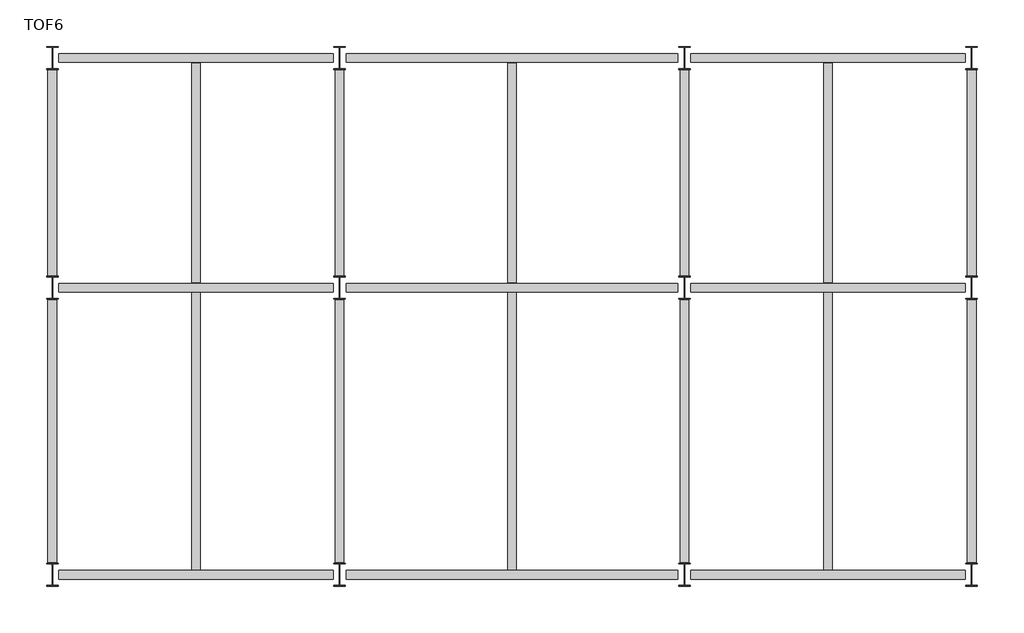
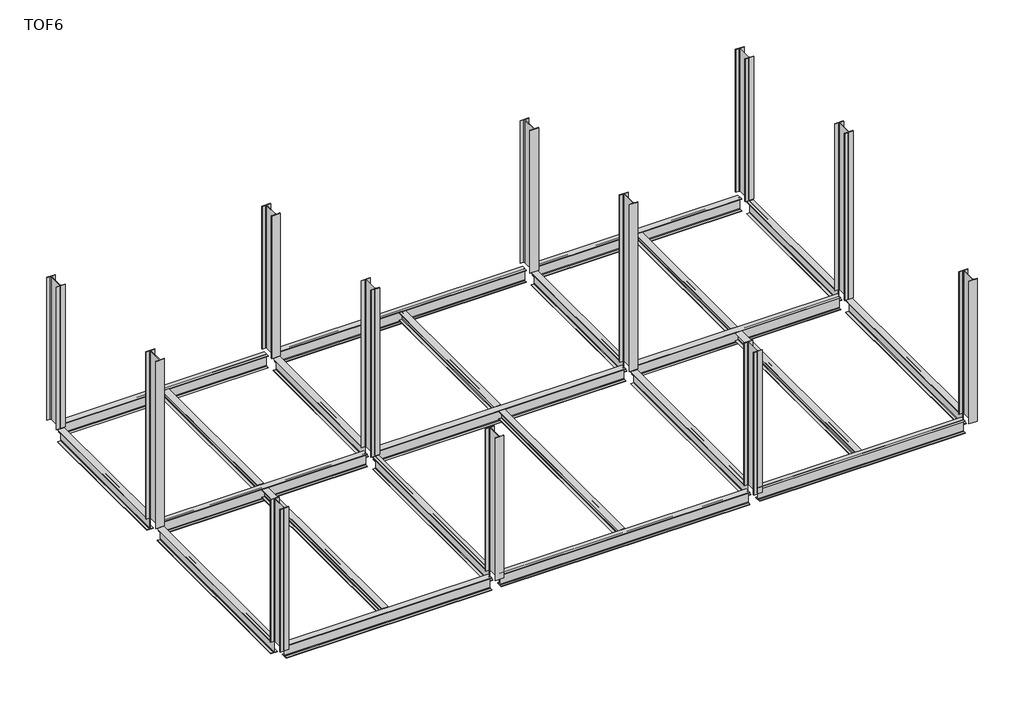
# One storey: 23 beams, 12 columns.
"""IFC4 building model written with IfcOpenShell, lengths in millimetres."""

import ifcopenshell
import ifcopenshell.guid

model = None  # the IFC model being written
_history = None  # IfcOwnerHistory: only IFC2X3 demands one
_inside = {}  # id of a spatial element -> (the spatial element, [elements in it])
_under = {}  # id of a project, library or spatial element -> (it, [spatial elements below it])
_declared = {}  # id of a project -> (the project, [libraries it declares])
_typed = {}  # id of a type object -> (the type object, [elements of that type])
_made_of = {}  # id of a material, layer set ... -> (it, [elements and type objects made of it])


def new_model(schema):
    """Start an empty IFC model of exactly this schema.

    Asked for "IFC4X3", IfcOpenShell would pick the latest addendum, in which some entities
    have other attributes; the version numbers below select the first issue.
    IFC2X3 requires an IfcOwnerHistory on every rooted entity: one is made here for all.
    """
    global model, _history
    if schema == "IFC4X3":
        model = ifcopenshell.file(schema_version=(4, 3, 0, 0))
    else:
        model = ifcopenshell.file(schema=schema)
    _inside.clear()
    _under.clear()
    _declared.clear()
    _typed.clear()
    _made_of.clear()
    _history = None
    if model.schema == "IFC2X3":
        org = make("IfcOrganization", Name="unknown")
        user = make(
            "IfcPersonAndOrganization",
            ThePerson=make("IfcPerson", FamilyName="unknown"),
            TheOrganization=org,
        )
        app = make(
            "IfcApplication",
            ApplicationDeveloper=org,
            Version="unknown",
            ApplicationFullName="unknown",
            ApplicationIdentifier="unknown",
        )
        _history = make(
            "IfcOwnerHistory",
            OwningUser=user,
            OwningApplication=app,
            ChangeAction="ADDED",
            CreationDate=0,
        )
    return model


def make(cls, **values):
    """One entity of the class cls with the attributes given. An attribute that is None is left unset."""
    return model.create_entity(
        cls, **{name: value for name, value in values.items() if value is not None}
    )


def rooted(cls, **values):
    """An entity with a GlobalId (a new one), such as an element, a storey or a relation."""
    return make(cls, GlobalId=ifcopenshell.guid.new(), OwnerHistory=_history, **values)


def si_unit(unit_type, name, prefix=None):
    """IfcSIUnit, for example si_unit("LENGTHUNIT", "METRE", prefix="MILLI")."""
    return make("IfcSIUnit", UnitType=unit_type, Prefix=prefix, Name=name)


def assignment(units):
    """IfcUnitAssignment: the units of a project."""
    return None if units is None else make("IfcUnitAssignment", Units=units)


def point(xyz):
    """IfcCartesianPoint."""
    return None if xyz is None else make("IfcCartesianPoint", Coordinates=xyz)


def direction(xyz):
    """IfcDirection."""
    return None if xyz is None else make("IfcDirection", DirectionRatios=xyz)


def frame(location, z_axis=None, x_axis=None):
    """IfcAxis2Placement3D, a coordinate frame: its origin and axes. An axis left out is left unset."""
    return make(
        "IfcAxis2Placement3D",
        Location=point(location),
        Axis=direction(z_axis),
        RefDirection=direction(x_axis),
    )


def frame_2d(location, x_axis=None):
    """IfcAxis2Placement2D, a coordinate frame in the plane: its origin and x axis."""
    return make(
        "IfcAxis2Placement2D", Location=point(location), RefDirection=direction(x_axis)
    )


def origin():
    """The frame at (0, 0, 0) with its axes left unset."""
    return frame((0.0, 0.0, 0.0))


def place(relative_to, where):
    """IfcLocalPlacement: puts the frame where relative to a parent placement (None: the world)."""
    return make(
        "IfcLocalPlacement", PlacementRelTo=relative_to, RelativePlacement=where
    )


def context(
    kind, dimensions, precision=None, world=None, true_north=None, identifier=None
):
    """IfcGeometricRepresentationContext, for example the 3D "Model" context."""
    return make(
        "IfcGeometricRepresentationContext",
        ContextIdentifier=identifier,
        ContextType=kind,
        CoordinateSpaceDimension=dimensions,
        Precision=precision,
        WorldCoordinateSystem=world,
        TrueNorth=true_north,
    )


def project(units=None, contexts=None):
    """IfcProject with its units and contexts."""
    return rooted(
        "IfcProject",
        Name="project",
        RepresentationContexts=contexts,
        UnitsInContext=assignment(units),
    )


def spatial(cls, under=None, at=None, **own):
    """A site, building, storey or space (cls), placed at a placement, below another one or the project."""
    s = rooted(cls, ObjectPlacement=at, **own)
    if under is not None:
        _under.setdefault(under.id(), (under, []))[1].append(s)
    return s


def polyline(points):
    """IfcPolyline through the points."""
    return make("IfcPolyline", Points=[point(p) for p in points])


def circle_curve(where, radius):
    """IfcCircle in the frame where."""
    return make("IfcCircle", Position=where, Radius=radius)


def trimmed(basis, trim1, trim2, sense, master):
    """IfcTrimmedCurve: the piece of a basis curve between two trims."""
    return make(
        "IfcTrimmedCurve",
        BasisCurve=basis,
        Trim1=trim1,
        Trim2=trim2,
        SenseAgreement=sense,
        MasterRepresentation=master,
    )


def segment(curve, same_sense, transition):
    """IfcCompositeCurveSegment."""
    return make(
        "IfcCompositeCurveSegment",
        Transition=transition,
        SameSense=same_sense,
        ParentCurve=curve,
    )


def composite_curve(segments, self_intersect=None):
    """IfcCompositeCurve: segments joined end to end."""
    return make("IfcCompositeCurve", Segments=segments, SelfIntersect=self_intersect)


def outline(outer, holes=None, kind="AREA"):
    """IfcArbitraryClosedProfileDef: a profile drawn as a closed curve; with holes, ...WithVoids."""
    if holes is None:
        return make("IfcArbitraryClosedProfileDef", ProfileType=kind, OuterCurve=outer)
    return make(
        "IfcArbitraryProfileDefWithVoids",
        ProfileType=kind,
        OuterCurve=outer,
        InnerCurves=holes,
    )


def extrude(swept, where, along, depth):
    """IfcExtrudedAreaSolid: the profile swept, set in the frame where, extruded along a direction by depth."""
    return make(
        "IfcExtrudedAreaSolid",
        SweptArea=swept,
        Position=where,
        ExtrudedDirection=direction(along),
        Depth=depth,
    )


def shape(context_of_items, identifier, shape_type, items):
    """IfcShapeRepresentation: the items that make up one representation, for example the "Body"."""
    return make(
        "IfcShapeRepresentation",
        ContextOfItems=context_of_items,
        RepresentationIdentifier=identifier,
        RepresentationType=shape_type,
        Items=items,
    )


def source(mapping_origin, context_of_items, identifier, shape_type, items):
    """IfcRepresentationMap: a shape defined once, which mapped items show again and again."""
    return make(
        "IfcRepresentationMap",
        MappingOrigin=mapping_origin,
        MappedRepresentation=shape(context_of_items, identifier, shape_type, items),
    )


def transform(
    local_origin,
    x_axis=None,
    y_axis=None,
    z_axis=None,
    scale=None,
    scale2=None,
    scale3=None,
    uniform=True,
):
    """IfcCartesianTransformationOperator3D, or its non-uniform kind. x_axis, y_axis, z_axis: its Axis1, 2, 3."""
    if uniform:
        return make(
            "IfcCartesianTransformationOperator3D",
            Axis1=direction(x_axis),
            Axis2=direction(y_axis),
            LocalOrigin=point(local_origin),
            Scale=scale,
            Axis3=direction(z_axis),
        )
    return make(
        "IfcCartesianTransformationOperator3DnonUniform",
        Axis1=direction(x_axis),
        Axis2=direction(y_axis),
        LocalOrigin=point(local_origin),
        Scale=scale,
        Axis3=direction(z_axis),
        Scale2=scale2,
        Scale3=scale3,
    )


def mapped(mapping_source, mapping_target):
    """IfcMappedItem: shows the shape of a source again, moved by a transform."""
    return make(
        "IfcMappedItem", MappingSource=mapping_source, MappingTarget=mapping_target
    )


def made_of(thing, what):
    """Note that an element or type object is made of a material, layer set ...; save() writes the relation."""
    if what is not None:
        _made_of.setdefault(what.id(), (what, []))[1].append(thing)
    return thing


def element(
    cls,
    number,
    at=None,
    inside=None,
    cuts=None,
    type_object=None,
    material=None,
    context=None,
    identifier="Body",
    shape_type=None,
    held_by="IfcProductDefinitionShape",
    body=None,
    shapes=None,
    **own,
):
    """One element of the class cls, such as IfcWall. Its Tag is "e" and its number.

    at: its placement. inside: the storey or other place that contains it. cuts: it is an
    opening in that element (IfcRelVoidsElement). A single representation is given by context,
    identifier, shape_type and body (its items); several are given by shapes. held_by: the class
    of the entity that holds the representations. save() writes the other relations.
    """
    e = rooted(cls, Tag="e%d" % number, ObjectPlacement=at, **own)
    if body is not None:
        shapes = [shape(context, identifier, shape_type, body)]
    if shapes is not None:
        e.Representation = make(held_by, Representations=shapes)
    if inside is not None:
        _inside.setdefault(inside.id(), (inside, []))[1].append(e)
    if cuts is not None:
        rooted(
            "IfcRelVoidsElement", RelatingBuildingElement=cuts, RelatedOpeningElement=e
        )
    if type_object is not None:
        _typed.setdefault(type_object.id(), (type_object, []))[1].append(e)
    return made_of(e, material)


def aggregate(whole, parts):
    """IfcRelAggregates: a whole, such as a stair, and the parts it consists of."""
    return rooted("IfcRelAggregates", RelatingObject=whole, RelatedObjects=parts)


def save(model, path):
    """Write the relations noted so far, then the file.

    IfcRelAggregates (storeys below a building ...), IfcRelContainedInSpatialStructure (elements
    in a storey), IfcRelDefinesByType, IfcRelAssociatesMaterial and IfcRelDeclares: one each for
    every whole, place, type object, material and project.
    """
    for whole, parts in _under.values():
        aggregate(whole, parts)
    for where, things in _inside.values():
        rooted(
            "IfcRelContainedInSpatialStructure",
            RelatedElements=things,
            RelatingStructure=where,
        )
    for kind, things in _typed.values():
        rooted("IfcRelDefinesByType", RelatedObjects=things, RelatingType=kind)
    for what, things in _made_of.values():
        rooted("IfcRelAssociatesMaterial", RelatedObjects=things, RelatingMaterial=what)
    for by, libraries in _declared.values():
        rooted("IfcRelDeclares", RelatingContext=by, RelatedDefinitions=libraries)
    model.write(path)


def beam_a4a24592(model_context):
    return source(origin(), model_context, "Body", "SweptSolid", [
        extrude(outline(composite_curve([segment(polyline([(75.0, -141.0), (75.0, -150.0), (-75.0, -150.0), (-75.0, -141.0), (-16.25, -141.0)]), True, "CONTINUOUS"), segment(trimmed(circle_curve(frame_2d((-16.25, -128.0)), 13.0), [point((-16.25, -141.0))], [point((-3.25, -128.0))], True, "CARTESIAN"), True, "CONTINUOUS"), segment(polyline([(-3.25, -128.0), (-3.25, 128.0)]), True, "CONTINUOUS"), segment(trimmed(circle_curve(frame_2d((-16.25, 128.0)), 13.0), [point((-3.25, 128.0))], [point((-16.25, 141.0))], True, "CARTESIAN"), True, "CONTINUOUS"), segment(polyline([(-16.25, 141.0), (-75.0, 141.0), (-75.0, 150.0), (75.0, 150.0), (75.0, 141.0), (16.25, 141.0)]), True, "CONTINUOUS"), segment(trimmed(circle_curve(frame_2d((16.25, 128.0)), 13.0), [point((16.25, 141.0))], [point((3.25, 128.0))], True, "CARTESIAN"), True, "CONTINUOUS"), segment(polyline([(3.25, 128.0), (3.25, -128.0)]), True, "CONTINUOUS"), segment(trimmed(circle_curve(frame_2d((16.25, -128.0)), 13.0), [point((3.25, -128.0))], [point((16.25, -141.0))], True, "CARTESIAN"), True, "CONTINUOUS"), segment(polyline([(16.25, -141.0), (75.0, -141.0)]), True, "CONTINUOUS")], self_intersect=False)), frame((-2387.3, 0.0, 0.0), z_axis=(1.0, 0.0, 0.0), x_axis=(0.0, 1.0, 0.0)), (0.0, 0.0, 1.0), 4774.6),
    ])


def beam_98be4253(model_context):
    return source(origin(), model_context, "Body", "SweptSolid", [
        extrude(outline(composite_curve([segment(polyline([(75.0, -141.0), (75.0, -150.0), (-75.0, -150.0), (-75.0, -141.0), (-16.25, -141.0)]), True, "CONTINUOUS"), segment(trimmed(circle_curve(frame_2d((-16.25, -128.0)), 13.0), [point((-16.25, -141.0))], [point((-3.25, -128.0))], True, "CARTESIAN"), True, "CONTINUOUS"), segment(polyline([(-3.25, -128.0), (-3.25, 128.0)]), True, "CONTINUOUS"), segment(trimmed(circle_curve(frame_2d((-16.25, 128.0)), 13.0), [point((-3.25, 128.0))], [point((-16.25, 141.0))], True, "CARTESIAN"), True, "CONTINUOUS"), segment(polyline([(-16.25, 141.0), (-75.0, 141.0), (-75.0, 150.0), (75.0, 150.0), (75.0, 141.0), (16.25, 141.0)]), True, "CONTINUOUS"), segment(trimmed(circle_curve(frame_2d((16.25, 128.0)), 13.0), [point((16.25, 141.0))], [point((3.25, 128.0))], True, "CARTESIAN"), True, "CONTINUOUS"), segment(polyline([(3.25, 128.0), (3.25, -128.0)]), True, "CONTINUOUS"), segment(trimmed(circle_curve(frame_2d((16.25, -128.0)), 13.0), [point((3.25, -128.0))], [point((16.25, -141.0))], True, "CARTESIAN"), True, "CONTINUOUS"), segment(polyline([(16.25, -141.0), (75.0, -141.0)]), True, "CONTINUOUS")], self_intersect=False)), frame((-2887.3, 0.0, 0.0), z_axis=(1.0, 0.0, 0.0), x_axis=(0.0, 1.0, 0.0)), (0.0, 0.0, 1.0), 5774.6),
    ])


def beam_4b5297f3(model_context):
    return source(origin(), model_context, "Body", "SweptSolid", [
        extrude(outline(composite_curve([segment(polyline([(75.0, -141.0), (75.0, -150.0), (-75.0, -150.0), (-75.0, -141.0), (-16.25, -141.0)]), True, "CONTINUOUS"), segment(trimmed(circle_curve(frame_2d((-16.25, -128.0)), 13.0), [point((-16.25, -141.0))], [point((-3.25, -128.0))], True, "CARTESIAN"), True, "CONTINUOUS"), segment(polyline([(-3.25, -128.0), (-3.25, 128.0)]), True, "CONTINUOUS"), segment(trimmed(circle_curve(frame_2d((-16.25, 128.0)), 13.0), [point((-3.25, 128.0))], [point((-16.25, 141.0))], True, "CARTESIAN"), True, "CONTINUOUS"), segment(polyline([(-16.25, 141.0), (-75.0, 141.0), (-75.0, 150.0), (75.0, 150.0), (75.0, 141.0), (16.25, 141.0)]), True, "CONTINUOUS"), segment(trimmed(circle_curve(frame_2d((16.25, 128.0)), 13.0), [point((16.25, 141.0))], [point((3.25, 128.0))], True, "CARTESIAN"), True, "CONTINUOUS"), segment(polyline([(3.25, 128.0), (3.25, -128.0)]), True, "CONTINUOUS"), segment(trimmed(circle_curve(frame_2d((16.25, -128.0)), 13.0), [point((3.25, -128.0))], [point((16.25, -141.0))], True, "CARTESIAN"), True, "CONTINUOUS"), segment(polyline([(16.25, -141.0), (75.0, -141.0)]), True, "CONTINUOUS")], self_intersect=False)), frame((-2287.3, 0.0, 0.0), z_axis=(1.0, 0.0, 0.0), x_axis=(0.0, 1.0, 0.0)), (0.0, 0.0, 1.0), 4574.6),
    ])


def beam_dad7a266(model_context):
    return source(origin(), model_context, "Body", "SweptSolid", [
        extrude(outline(composite_curve([segment(polyline([(75.0, -141.0), (75.0, -150.0), (-75.0, -150.0), (-75.0, -141.0), (-16.25, -141.0)]), True, "CONTINUOUS"), segment(trimmed(circle_curve(frame_2d((-16.25, -128.0)), 13.0), [point((-16.25, -141.0))], [point((-3.25, -128.0))], True, "CARTESIAN"), True, "CONTINUOUS"), segment(polyline([(-3.25, -128.0), (-3.25, 128.0)]), True, "CONTINUOUS"), segment(trimmed(circle_curve(frame_2d((-16.25, 128.0)), 13.0), [point((-3.25, 128.0))], [point((-16.25, 141.0))], True, "CARTESIAN"), True, "CONTINUOUS"), segment(polyline([(-16.25, 141.0), (-75.0, 141.0), (-75.0, 150.0), (75.0, 150.0), (75.0, 141.0), (16.25, 141.0)]), True, "CONTINUOUS"), segment(trimmed(circle_curve(frame_2d((16.25, 128.0)), 13.0), [point((16.25, 141.0))], [point((3.25, 128.0))], True, "CARTESIAN"), True, "CONTINUOUS"), segment(polyline([(3.25, 128.0), (3.25, -128.0)]), True, "CONTINUOUS"), segment(trimmed(circle_curve(frame_2d((16.25, -128.0)), 13.0), [point((3.25, -128.0))], [point((16.25, -141.0))], True, "CARTESIAN"), True, "CONTINUOUS"), segment(polyline([(16.25, -141.0), (75.0, -141.0)]), True, "CONTINUOUS")], self_intersect=False)), frame((-1787.3, 0.0, 0.0), z_axis=(1.0, 0.0, 0.0), x_axis=(0.0, 1.0, 0.0)), (0.0, 0.0, 1.0), 3574.6),
    ])


def beam_719db1ac(model_context):
    return source(origin(), model_context, "Body", "SweptSolid", [
        extrude(outline(composite_curve([segment(polyline([(75.0, -88.0), (75.0, -97.0), (-75.0, -97.0), (-75.0, -88.0), (-16.0, -88.0)]), True, "CONTINUOUS"), segment(trimmed(circle_curve(frame_2d((-16.0, -75.0)), 13.0), [point((-16.0, -88.0))], [point((-3.0, -75.0))], True, "CARTESIAN"), True, "CONTINUOUS"), segment(polyline([(-3.0, -75.0), (-3.0, 75.0)]), True, "CONTINUOUS"), segment(trimmed(circle_curve(frame_2d((-16.0, 75.0)), 13.0), [point((-3.0, 75.0))], [point((-16.0, 88.0))], True, "CARTESIAN"), True, "CONTINUOUS"), segment(polyline([(-16.0, 88.0), (-75.0, 88.0), (-75.0, 97.0), (75.0, 97.0), (75.0, 88.0), (16.0, 88.0)]), True, "CONTINUOUS"), segment(trimmed(circle_curve(frame_2d((16.0, 75.0)), 13.0), [point((16.0, 88.0))], [point((3.0, 75.0))], True, "CARTESIAN"), True, "CONTINUOUS"), segment(polyline([(3.0, 75.0), (3.0, -75.0)]), True, "CONTINUOUS"), segment(trimmed(circle_curve(frame_2d((16.0, -75.0)), 13.0), [point((3.0, -75.0))], [point((16.0, -88.0))], True, "CARTESIAN"), True, "CONTINUOUS"), segment(polyline([(16.0, -88.0), (75.0, -88.0)]), True, "CONTINUOUS")], self_intersect=False)), frame((-2412.3, 0.0, 0.0), z_axis=(1.0, 0.0, 0.0), x_axis=(0.0, 1.0, 0.0)), (0.0, 0.0, 1.0), 4824.6),
    ])


def beam_533db150(model_context):
    return source(origin(), model_context, "Body", "SweptSolid", [
        extrude(outline(composite_curve([segment(polyline([(75.0, -88.0), (75.0, -97.0), (-75.0, -97.0), (-75.0, -88.0), (-16.0, -88.0)]), True, "CONTINUOUS"), segment(trimmed(circle_curve(frame_2d((-16.0, -75.0)), 13.0), [point((-16.0, -88.0))], [point((-3.0, -75.0))], True, "CARTESIAN"), True, "CONTINUOUS"), segment(polyline([(-3.0, -75.0), (-3.0, 75.0)]), True, "CONTINUOUS"), segment(trimmed(circle_curve(frame_2d((-16.0, 75.0)), 13.0), [point((-3.0, 75.0))], [point((-16.0, 88.0))], True, "CARTESIAN"), True, "CONTINUOUS"), segment(polyline([(-16.0, 88.0), (-75.0, 88.0), (-75.0, 97.0), (75.0, 97.0), (75.0, 88.0), (16.0, 88.0)]), True, "CONTINUOUS"), segment(trimmed(circle_curve(frame_2d((16.0, 75.0)), 13.0), [point((16.0, 88.0))], [point((3.0, 75.0))], True, "CARTESIAN"), True, "CONTINUOUS"), segment(polyline([(3.0, 75.0), (3.0, -75.0)]), True, "CONTINUOUS"), segment(trimmed(circle_curve(frame_2d((16.0, -75.0)), 13.0), [point((3.0, -75.0))], [point((16.0, -88.0))], True, "CARTESIAN"), True, "CONTINUOUS"), segment(polyline([(16.0, -88.0), (75.0, -88.0)]), True, "CONTINUOUS")], self_intersect=False)), frame((-1912.3, 0.0, 0.0), z_axis=(1.0, 0.0, 0.0), x_axis=(0.0, 1.0, 0.0)), (0.0, 0.0, 1.0), 3824.6),
    ])


model = new_model("IFC4")

# Units and contexts
model_context = context("Model", 3, world=origin())
ifc_project = project(units=[si_unit("LENGTHUNIT", "METRE", prefix="MILLI")], contexts=[model_context])

# Site, building, storey
site = spatial("IfcSite", under=ifc_project)
building = spatial("IfcBuilding", under=site)
storey = spatial("IfcBuildingStorey", under=building, Name="TOF6", Elevation=9000.0)

# Beams
placement = place(None, origin())
beam_shape = beam_a4a24592(model_context)
element("IfcBeam", 1, ObjectType="0912_Steel Framing_H-KSD3502 : H_SB_AR_S02_H-300x150x6.5x9_Stair", at=placement, inside=storey, context=model_context, shape_type="MappedRepresentation", body=[
    mapped(beam_shape, transform((2500.0, 0.0, 8850.0), x_axis=(1.0, 0.0, 0.0), y_axis=(0.0, 1.0, 0.0), z_axis=(0.0, 0.0, 1.0))),
])
element("IfcBeam", 2, ObjectType="0912_Steel Framing_H-KSD3502 : H_SB_AR_S02_H-300x150x6.5x9_Stair", at=placement, inside=storey, context=model_context, shape_type="MappedRepresentation", body=[
    mapped(beam_shape, transform((13500.0, 0.0, 8850.0), x_axis=(1.0, 0.0, 0.0), y_axis=(0.0, 1.0, 0.0), z_axis=(0.0, 0.0, 1.0))),
])
element("IfcBeam", 3, ObjectType="0912_Steel Framing_H-KSD3502 : H_SB_AR_S02_H-300x150x6.5x9_Stair", at=placement, inside=storey, context=model_context, shape_type="MappedRepresentation", body=[
    mapped(beam_shape, transform((2500.0, 5000.0, 8850.0), x_axis=(1.0, 0.0, 0.0), y_axis=(0.0, 1.0, 0.0), z_axis=(0.0, 0.0, 1.0))),
])
element("IfcBeam", 4, ObjectType="0912_Steel Framing_H-KSD3502 : H_SB_AR_S02_H-300x150x6.5x9_Stair", at=placement, inside=storey, context=model_context, shape_type="MappedRepresentation", body=[
    mapped(beam_shape, transform((13500.0, 5000.0, 8850.0), x_axis=(1.0, 0.0, 0.0), y_axis=(0.0, 1.0, 0.0), z_axis=(0.0, 0.0, 1.0))),
])
element("IfcBeam", 5, ObjectType="0912_Steel Framing_H-KSD3502 : H_SB_AR_S02_H-300x150x6.5x9_Stair", at=placement, inside=storey, context=model_context, shape_type="MappedRepresentation", body=[
    mapped(beam_shape, transform((2500.0, 9000.0, 8850.0), x_axis=(1.0, 0.0, 0.0), y_axis=(0.0, 1.0, 0.0), z_axis=(0.0, 0.0, 1.0))),
])
element("IfcBeam", 6, ObjectType="0912_Steel Framing_H-KSD3502 : H_SB_AR_S02_H-300x150x6.5x9_Stair", at=placement, inside=storey, context=model_context, shape_type="MappedRepresentation", body=[
    mapped(beam_shape, transform((13500.0, 9000.0, 8850.0), x_axis=(1.0, 0.0, 0.0), y_axis=(0.0, 1.0, 0.0), z_axis=(0.0, 0.0, 1.0))),
])
beam_2_shape = beam_98be4253(model_context)
element("IfcBeam", 7, ObjectType="0912_Steel Framing_H-KSD3502 : H_SB_AR_S02_H-300x150x6.5x9_Stair", at=placement, inside=storey, context=model_context, shape_type="MappedRepresentation", body=[
    mapped(beam_2_shape, transform((8000.0, 0.0, 8850.0), x_axis=(1.0, 0.0, 0.0), y_axis=(0.0, 1.0, 0.0), z_axis=(0.0, 0.0, 1.0))),
])
element("IfcBeam", 8, ObjectType="0912_Steel Framing_H-KSD3502 : H_SB_AR_S02_H-300x150x6.5x9_Stair", at=placement, inside=storey, context=model_context, shape_type="MappedRepresentation", body=[
    mapped(beam_2_shape, transform((8000.0, 5000.0, 8850.0), x_axis=(1.0, 0.0, 0.0), y_axis=(0.0, 1.0, 0.0), z_axis=(0.0, 0.0, 1.0))),
])
element("IfcBeam", 9, ObjectType="0912_Steel Framing_H-KSD3502 : H_SB_AR_S02_H-300x150x6.5x9_Stair", at=placement, inside=storey, context=model_context, shape_type="MappedRepresentation", body=[
    mapped(beam_2_shape, transform((8000.0, 9000.0, 8850.0), x_axis=(1.0, 0.0, 0.0), y_axis=(0.0, 1.0, 0.0), z_axis=(0.0, 0.0, 1.0))),
])
beam_3_shape = beam_4b5297f3(model_context)
element("IfcBeam", 10, ObjectType="0912_Steel Framing_H-KSD3502 : H_SB_AR_S02_H-300x150x6.5x9_Stair", at=placement, inside=storey, context=model_context, shape_type="MappedRepresentation", body=[
    mapped(beam_3_shape, transform((0.0, 2500.0, 8850.0), x_axis=(0.0, 1.0, 0.0), y_axis=(-1.0, 0.0, 0.0), z_axis=(0.0, 0.0, 1.0))),
])
element("IfcBeam", 11, ObjectType="0912_Steel Framing_H-KSD3502 : H_SB_AR_S02_H-300x150x6.5x9_Stair", at=placement, inside=storey, context=model_context, shape_type="MappedRepresentation", body=[
    mapped(beam_3_shape, transform((5000.0, 2500.0, 8850.0), x_axis=(0.0, 1.0, 0.0), y_axis=(-1.0, 0.0, 0.0), z_axis=(0.0, 0.0, 1.0))),
])
element("IfcBeam", 12, ObjectType="0912_Steel Framing_H-KSD3502 : H_SB_AR_S02_H-300x150x6.5x9_Stair", at=placement, inside=storey, context=model_context, shape_type="MappedRepresentation", body=[
    mapped(beam_3_shape, transform((11000.0, 2500.0, 8850.0), x_axis=(0.0, 1.0, 0.0), y_axis=(-1.0, 0.0, 0.0), z_axis=(0.0, 0.0, 1.0))),
])
element("IfcBeam", 13, ObjectType="0912_Steel Framing_H-KSD3502 : H_SB_AR_S02_H-300x150x6.5x9_Stair", at=placement, inside=storey, context=model_context, shape_type="MappedRepresentation", body=[
    mapped(beam_3_shape, transform((16000.0, 2500.0, 8850.0), x_axis=(0.0, 1.0, 0.0), y_axis=(-1.0, 0.0, 0.0), z_axis=(0.0, 0.0, 1.0))),
])
beam_4_shape = beam_dad7a266(model_context)
element("IfcBeam", 14, ObjectType="0912_Steel Framing_H-KSD3502 : H_SB_AR_S02_H-300x150x6.5x9_Stair", at=placement, inside=storey, context=model_context, shape_type="MappedRepresentation", body=[
    mapped(beam_4_shape, transform((0.0, 7000.0, 8850.0), x_axis=(0.0, 1.0, 0.0), y_axis=(-1.0, 0.0, 0.0), z_axis=(0.0, 0.0, 1.0))),
])
element("IfcBeam", 15, ObjectType="0912_Steel Framing_H-KSD3502 : H_SB_AR_S02_H-300x150x6.5x9_Stair", at=placement, inside=storey, context=model_context, shape_type="MappedRepresentation", body=[
    mapped(beam_4_shape, transform((5000.0, 7000.0, 8850.0), x_axis=(0.0, 1.0, 0.0), y_axis=(-1.0, 0.0, 0.0), z_axis=(0.0, 0.0, 1.0))),
])
element("IfcBeam", 16, ObjectType="0912_Steel Framing_H-KSD3502 : H_SB_AR_S02_H-300x150x6.5x9_Stair", at=placement, inside=storey, context=model_context, shape_type="MappedRepresentation", body=[
    mapped(beam_4_shape, transform((11000.0, 7000.0, 8850.0), x_axis=(0.0, 1.0, 0.0), y_axis=(-1.0, 0.0, 0.0), z_axis=(0.0, 0.0, 1.0))),
])
element("IfcBeam", 17, ObjectType="0912_Steel Framing_H-KSD3502 : H_SB_AR_S02_H-300x150x6.5x9_Stair", at=placement, inside=storey, context=model_context, shape_type="MappedRepresentation", body=[
    mapped(beam_4_shape, transform((16000.0, 7000.0, 8850.0), x_axis=(0.0, 1.0, 0.0), y_axis=(-1.0, 0.0, 0.0), z_axis=(0.0, 0.0, 1.0))),
])
beam_5_shape = beam_719db1ac(model_context)
element("IfcBeam", 18, ObjectType="0912_Steel Framing_H-KSD3502 : H_SB_AR_S02_H-194x150x6x9_Platform", at=placement, inside=storey, context=model_context, shape_type="MappedRepresentation", body=[
    mapped(beam_5_shape, transform((2500.0, 2500.0, 8903.0), x_axis=(0.0, 1.0, 0.0), y_axis=(-1.0, 0.0, 0.0), z_axis=(0.0, 0.0, 1.0))),
])
element("IfcBeam", 19, ObjectType="0912_Steel Framing_H-KSD3502 : H_SB_AR_S02_H-194x150x6x9_Platform", at=placement, inside=storey, context=model_context, shape_type="MappedRepresentation", body=[
    mapped(beam_5_shape, transform((8000.0, 2500.0, 8903.0), x_axis=(0.0, 1.0, 0.0), y_axis=(-1.0, 0.0, 0.0), z_axis=(0.0, 0.0, 1.0))),
])
element("IfcBeam", 20, ObjectType="0912_Steel Framing_H-KSD3502 : H_SB_AR_S02_H-194x150x6x9_Platform", at=placement, inside=storey, context=model_context, shape_type="MappedRepresentation", body=[
    mapped(beam_5_shape, transform((13500.0, 2500.0, 8903.0), x_axis=(0.0, 1.0, 0.0), y_axis=(-1.0, 0.0, 0.0), z_axis=(0.0, 0.0, 1.0))),
])
beam_6_shape = beam_533db150(model_context)
element("IfcBeam", 21, ObjectType="0912_Steel Framing_H-KSD3502 : H_SB_AR_S02_H-194x150x6x9_Platform", at=placement, inside=storey, context=model_context, shape_type="MappedRepresentation", body=[
    mapped(beam_6_shape, transform((2500.0, 7000.0, 8903.0), x_axis=(0.0, 1.0, 0.0), y_axis=(-1.0, 0.0, 0.0), z_axis=(0.0, 0.0, 1.0))),
])
element("IfcBeam", 22, ObjectType="0912_Steel Framing_H-KSD3502 : H_SB_AR_S02_H-194x150x6x9_Platform", at=placement, inside=storey, context=model_context, shape_type="MappedRepresentation", body=[
    mapped(beam_6_shape, transform((8000.0, 7000.0, 8903.0), x_axis=(0.0, 1.0, 0.0), y_axis=(-1.0, 0.0, 0.0), z_axis=(0.0, 0.0, 1.0))),
])
element("IfcBeam", 23, ObjectType="0912_Steel Framing_H-KSD3502 : H_SB_AR_S02_H-194x150x6x9_Platform", at=placement, inside=storey, context=model_context, shape_type="MappedRepresentation", body=[
    mapped(beam_6_shape, transform((13500.0, 7000.0, 8903.0), x_axis=(0.0, 1.0, 0.0), y_axis=(-1.0, 0.0, 0.0), z_axis=(0.0, 0.0, 1.0))),
])

# Columns
element("IfcColumn", 24, ObjectType="Steel Column_H_KSD3502 : H_SC_AR_S01_H-400x200x8x13", at=placement, inside=storey, context=model_context, shape_type="SweptSolid", body=[
    extrude(outline(composite_curve([segment(polyline([(100.0, 200.0), (100.0, 187.0), (20.0, 187.0)]), True, "CONTINUOUS"), segment(trimmed(circle_curve(frame_2d((20.0, 171.0)), 16.0), [point((20.0, 187.0))], [point((4.0, 171.0))], True, "CARTESIAN"), True, "CONTINUOUS"), segment(polyline([(4.0, 171.0), (4.0, -171.0)]), True, "CONTINUOUS"), segment(trimmed(circle_curve(frame_2d((20.0, -171.0)), 16.0), [point((4.0, -171.0))], [point((20.0, -187.0))], True, "CARTESIAN"), True, "CONTINUOUS"), segment(polyline([(20.0, -187.0), (100.0, -187.0), (100.0, -200.0), (-100.0, -200.0), (-100.0, -187.0), (-20.0, -187.0)]), True, "CONTINUOUS"), segment(trimmed(circle_curve(frame_2d((-20.0, -171.0)), 16.0), [point((-20.0, -187.0))], [point((-4.0, -171.0))], True, "CARTESIAN"), True, "CONTINUOUS"), segment(polyline([(-4.0, -171.0), (-4.0, 171.0)]), True, "CONTINUOUS"), segment(trimmed(circle_curve(frame_2d((-20.0, 171.0)), 16.0), [point((-4.0, 171.0))], [point((-20.0, 187.0))], True, "CARTESIAN"), True, "CONTINUOUS"), segment(polyline([(-20.0, 187.0), (-100.0, 187.0), (-100.0, 200.0), (100.0, 200.0)]), True, "CONTINUOUS")], self_intersect=False)), frame((0.0, 0.0, 9000.0), z_axis=(0.0, 0.0, 1.0), x_axis=(1.0, 0.0, 0.0)), (0.0, 0.0, 1.0), 3500.0),
])
element("IfcColumn", 25, ObjectType="Steel Column_H_KSD3502 : H_SC_AR_S01_H-400x200x8x13", at=placement, inside=storey, context=model_context, shape_type="SweptSolid", body=[
    extrude(outline(composite_curve([segment(polyline([(5100.0, 200.0), (5100.0, 187.0), (5020.0, 187.0)]), True, "CONTINUOUS"), segment(trimmed(circle_curve(frame_2d((5020.0, 171.0)), 16.0), [point((5020.0, 187.0))], [point((5004.0, 171.0))], True, "CARTESIAN"), True, "CONTINUOUS"), segment(polyline([(5004.0, 171.0), (5004.0, -171.0)]), True, "CONTINUOUS"), segment(trimmed(circle_curve(frame_2d((5020.0, -171.0)), 16.0), [point((5004.0, -171.0))], [point((5020.0, -187.0))], True, "CARTESIAN"), True, "CONTINUOUS"), segment(polyline([(5020.0, -187.0), (5100.0, -187.0), (5100.0, -200.0), (4900.0, -200.0), (4900.0, -187.0), (4980.0, -187.0)]), True, "CONTINUOUS"), segment(trimmed(circle_curve(frame_2d((4980.0, -171.0)), 16.0), [point((4980.0, -187.0))], [point((4996.0, -171.0))], True, "CARTESIAN"), True, "CONTINUOUS"), segment(polyline([(4996.0, -171.0), (4996.0, 171.0)]), True, "CONTINUOUS"), segment(trimmed(circle_curve(frame_2d((4980.0, 171.0)), 16.0), [point((4996.0, 171.0))], [point((4980.0, 187.0))], True, "CARTESIAN"), True, "CONTINUOUS"), segment(polyline([(4980.0, 187.0), (4900.0, 187.0), (4900.0, 200.0), (5100.0, 200.0)]), True, "CONTINUOUS")], self_intersect=False)), frame((0.0, 0.0, 9000.0), z_axis=(0.0, 0.0, 1.0), x_axis=(1.0, 0.0, 0.0)), (0.0, 0.0, 1.0), 3500.0),
])
element("IfcColumn", 26, ObjectType="Steel Column_H_KSD3502 : H_SC_AR_S01_H-400x200x8x13", at=placement, inside=storey, context=model_context, shape_type="SweptSolid", body=[
    extrude(outline(composite_curve([segment(polyline([(11100.0, 200.0), (11100.0, 187.0), (11020.0, 187.0)]), True, "CONTINUOUS"), segment(trimmed(circle_curve(frame_2d((11020.0, 171.0)), 16.0), [point((11020.0, 187.0))], [point((11004.0, 171.0))], True, "CARTESIAN"), True, "CONTINUOUS"), segment(polyline([(11004.0, 171.0), (11004.0, -171.0)]), True, "CONTINUOUS"), segment(trimmed(circle_curve(frame_2d((11020.0, -171.0)), 16.0), [point((11004.0, -171.0))], [point((11020.0, -187.0))], True, "CARTESIAN"), True, "CONTINUOUS"), segment(polyline([(11020.0, -187.0), (11100.0, -187.0), (11100.0, -200.0), (10900.0, -200.0), (10900.0, -187.0), (10980.0, -187.0)]), True, "CONTINUOUS"), segment(trimmed(circle_curve(frame_2d((10980.0, -171.0)), 16.0), [point((10980.0, -187.0))], [point((10996.0, -171.0))], True, "CARTESIAN"), True, "CONTINUOUS"), segment(polyline([(10996.0, -171.0), (10996.0, 171.0)]), True, "CONTINUOUS"), segment(trimmed(circle_curve(frame_2d((10980.0, 171.0)), 16.0), [point((10996.0, 171.0))], [point((10980.0, 187.0))], True, "CARTESIAN"), True, "CONTINUOUS"), segment(polyline([(10980.0, 187.0), (10900.0, 187.0), (10900.0, 200.0), (11100.0, 200.0)]), True, "CONTINUOUS")], self_intersect=False)), frame((0.0, 0.0, 9000.0), z_axis=(0.0, 0.0, 1.0), x_axis=(1.0, 0.0, 0.0)), (0.0, 0.0, 1.0), 3500.0),
])
element("IfcColumn", 27, ObjectType="Steel Column_H_KSD3502 : H_SC_AR_S01_H-400x200x8x13", at=placement, inside=storey, context=model_context, shape_type="SweptSolid", body=[
    extrude(outline(composite_curve([segment(polyline([(16100.0, 200.0), (16100.0, 187.0), (16020.0, 187.0)]), True, "CONTINUOUS"), segment(trimmed(circle_curve(frame_2d((16020.0, 171.0)), 16.0), [point((16020.0, 187.0))], [point((16004.0, 171.0))], True, "CARTESIAN"), True, "CONTINUOUS"), segment(polyline([(16004.0, 171.0), (16004.0, -171.0)]), True, "CONTINUOUS"), segment(trimmed(circle_curve(frame_2d((16020.0, -171.0)), 16.0), [point((16004.0, -171.0))], [point((16020.0, -187.0))], True, "CARTESIAN"), True, "CONTINUOUS"), segment(polyline([(16020.0, -187.0), (16100.0, -187.0), (16100.0, -200.0), (15900.0, -200.0), (15900.0, -187.0), (15980.0, -187.0)]), True, "CONTINUOUS"), segment(trimmed(circle_curve(frame_2d((15980.0, -171.0)), 16.0), [point((15980.0, -187.0))], [point((15996.0, -171.0))], True, "CARTESIAN"), True, "CONTINUOUS"), segment(polyline([(15996.0, -171.0), (15996.0, 171.0)]), True, "CONTINUOUS"), segment(trimmed(circle_curve(frame_2d((15980.0, 171.0)), 16.0), [point((15996.0, 171.0))], [point((15980.0, 187.0))], True, "CARTESIAN"), True, "CONTINUOUS"), segment(polyline([(15980.0, 187.0), (15900.0, 187.0), (15900.0, 200.0), (16100.0, 200.0)]), True, "CONTINUOUS")], self_intersect=False)), frame((0.0, 0.0, 9000.0), z_axis=(0.0, 0.0, 1.0), x_axis=(1.0, 0.0, 0.0)), (0.0, 0.0, 1.0), 3500.0),
])
element("IfcColumn", 28, ObjectType="Steel Column_H_KSD3502 : H_SC_AR_S01_H-400x200x8x13", at=placement, inside=storey, context=model_context, shape_type="SweptSolid", body=[
    extrude(outline(composite_curve([segment(polyline([(100.0, 5200.0), (100.0, 5187.0), (20.0, 5187.0)]), True, "CONTINUOUS"), segment(trimmed(circle_curve(frame_2d((20.0, 5171.0)), 16.0), [point((20.0, 5187.0))], [point((4.0, 5171.0))], True, "CARTESIAN"), True, "CONTINUOUS"), segment(polyline([(4.0, 5171.0), (4.0, 4829.0)]), True, "CONTINUOUS"), segment(trimmed(circle_curve(frame_2d((20.0, 4829.0)), 16.0), [point((4.0, 4829.0))], [point((20.0, 4813.0))], True, "CARTESIAN"), True, "CONTINUOUS"), segment(polyline([(20.0, 4813.0), (100.0, 4813.0), (100.0, 4800.0), (-100.0, 4800.0), (-100.0, 4813.0), (-20.0, 4813.0)]), True, "CONTINUOUS"), segment(trimmed(circle_curve(frame_2d((-20.0, 4829.0)), 16.0), [point((-20.0, 4813.0))], [point((-4.0, 4829.0))], True, "CARTESIAN"), True, "CONTINUOUS"), segment(polyline([(-4.0, 4829.0), (-4.0, 5171.0)]), True, "CONTINUOUS"), segment(trimmed(circle_curve(frame_2d((-20.0, 5171.0)), 16.0), [point((-4.0, 5171.0))], [point((-20.0, 5187.0))], True, "CARTESIAN"), True, "CONTINUOUS"), segment(polyline([(-20.0, 5187.0), (-100.0, 5187.0), (-100.0, 5200.0), (100.0, 5200.0)]), True, "CONTINUOUS")], self_intersect=False)), frame((0.0, 0.0, 9000.0), z_axis=(0.0, 0.0, 1.0), x_axis=(1.0, 0.0, 0.0)), (0.0, 0.0, 1.0), 4100.0),
])
element("IfcColumn", 29, ObjectType="Steel Column_H_KSD3502 : H_SC_AR_S01_H-400x200x8x13", at=placement, inside=storey, context=model_context, shape_type="SweptSolid", body=[
    extrude(outline(composite_curve([segment(polyline([(5100.0, 5200.0), (5100.0, 5187.0), (5020.0, 5187.0)]), True, "CONTINUOUS"), segment(trimmed(circle_curve(frame_2d((5020.0, 5171.0)), 16.0), [point((5020.0, 5187.0))], [point((5004.0, 5171.0))], True, "CARTESIAN"), True, "CONTINUOUS"), segment(polyline([(5004.0, 5171.0), (5004.0, 4829.0)]), True, "CONTINUOUS"), segment(trimmed(circle_curve(frame_2d((5020.0, 4829.0)), 16.0), [point((5004.0, 4829.0))], [point((5020.0, 4813.0))], True, "CARTESIAN"), True, "CONTINUOUS"), segment(polyline([(5020.0, 4813.0), (5100.0, 4813.0), (5100.0, 4800.0), (4900.0, 4800.0), (4900.0, 4813.0), (4980.0, 4813.0)]), True, "CONTINUOUS"), segment(trimmed(circle_curve(frame_2d((4980.0, 4829.0)), 16.0), [point((4980.0, 4813.0))], [point((4996.0, 4829.0))], True, "CARTESIAN"), True, "CONTINUOUS"), segment(polyline([(4996.0, 4829.0), (4996.0, 5171.0)]), True, "CONTINUOUS"), segment(trimmed(circle_curve(frame_2d((4980.0, 5171.0)), 16.0), [point((4996.0, 5171.0))], [point((4980.0, 5187.0))], True, "CARTESIAN"), True, "CONTINUOUS"), segment(polyline([(4980.0, 5187.0), (4900.0, 5187.0), (4900.0, 5200.0), (5100.0, 5200.0)]), True, "CONTINUOUS")], self_intersect=False)), frame((0.0, 0.0, 9000.0), z_axis=(0.0, 0.0, 1.0), x_axis=(1.0, 0.0, 0.0)), (0.0, 0.0, 1.0), 4100.0),
])
element("IfcColumn", 30, ObjectType="Steel Column_H_KSD3502 : H_SC_AR_S01_H-400x200x8x13", at=placement, inside=storey, context=model_context, shape_type="SweptSolid", body=[
    extrude(outline(composite_curve([segment(polyline([(11100.0, 5200.0), (11100.0, 5187.0), (11020.0, 5187.0)]), True, "CONTINUOUS"), segment(trimmed(circle_curve(frame_2d((11020.0, 5171.0)), 16.0), [point((11020.0, 5187.0))], [point((11004.0, 5171.0))], True, "CARTESIAN"), True, "CONTINUOUS"), segment(polyline([(11004.0, 5171.0), (11004.0, 4829.0)]), True, "CONTINUOUS"), segment(trimmed(circle_curve(frame_2d((11020.0, 4829.0)), 16.0), [point((11004.0, 4829.0))], [point((11020.0, 4813.0))], True, "CARTESIAN"), True, "CONTINUOUS"), segment(polyline([(11020.0, 4813.0), (11100.0, 4813.0), (11100.0, 4800.0), (10900.0, 4800.0), (10900.0, 4813.0), (10980.0, 4813.0)]), True, "CONTINUOUS"), segment(trimmed(circle_curve(frame_2d((10980.0, 4829.0)), 16.0), [point((10980.0, 4813.0))], [point((10996.0, 4829.0))], True, "CARTESIAN"), True, "CONTINUOUS"), segment(polyline([(10996.0, 4829.0), (10996.0, 5171.0)]), True, "CONTINUOUS"), segment(trimmed(circle_curve(frame_2d((10980.0, 5171.0)), 16.0), [point((10996.0, 5171.0))], [point((10980.0, 5187.0))], True, "CARTESIAN"), True, "CONTINUOUS"), segment(polyline([(10980.0, 5187.0), (10900.0, 5187.0), (10900.0, 5200.0), (11100.0, 5200.0)]), True, "CONTINUOUS")], self_intersect=False)), frame((0.0, 0.0, 9000.0), z_axis=(0.0, 0.0, 1.0), x_axis=(1.0, 0.0, 0.0)), (0.0, 0.0, 1.0), 4100.0),
])
element("IfcColumn", 31, ObjectType="Steel Column_H_KSD3502 : H_SC_AR_S01_H-400x200x8x13", at=placement, inside=storey, context=model_context, shape_type="SweptSolid", body=[
    extrude(outline(composite_curve([segment(polyline([(16100.0, 5200.0), (16100.0, 5187.0), (16020.0, 5187.0)]), True, "CONTINUOUS"), segment(trimmed(circle_curve(frame_2d((16020.0, 5171.0)), 16.0), [point((16020.0, 5187.0))], [point((16004.0, 5171.0))], True, "CARTESIAN"), True, "CONTINUOUS"), segment(polyline([(16004.0, 5171.0), (16004.0, 4829.0)]), True, "CONTINUOUS"), segment(trimmed(circle_curve(frame_2d((16020.0, 4829.0)), 16.0), [point((16004.0, 4829.0))], [point((16020.0, 4813.0))], True, "CARTESIAN"), True, "CONTINUOUS"), segment(polyline([(16020.0, 4813.0), (16100.0, 4813.0), (16100.0, 4800.0), (15900.0, 4800.0), (15900.0, 4813.0), (15980.0, 4813.0)]), True, "CONTINUOUS"), segment(trimmed(circle_curve(frame_2d((15980.0, 4829.0)), 16.0), [point((15980.0, 4813.0))], [point((15996.0, 4829.0))], True, "CARTESIAN"), True, "CONTINUOUS"), segment(polyline([(15996.0, 4829.0), (15996.0, 5171.0)]), True, "CONTINUOUS"), segment(trimmed(circle_curve(frame_2d((15980.0, 5171.0)), 16.0), [point((15996.0, 5171.0))], [point((15980.0, 5187.0))], True, "CARTESIAN"), True, "CONTINUOUS"), segment(polyline([(15980.0, 5187.0), (15900.0, 5187.0), (15900.0, 5200.0), (16100.0, 5200.0)]), True, "CONTINUOUS")], self_intersect=False)), frame((0.0, 0.0, 9000.0), z_axis=(0.0, 0.0, 1.0), x_axis=(1.0, 0.0, 0.0)), (0.0, 0.0, 1.0), 4100.0),
])
element("IfcColumn", 32, ObjectType="Steel Column_H_KSD3502 : H_SC_AR_S01_H-400x200x8x13", at=placement, inside=storey, context=model_context, shape_type="SweptSolid", body=[
    extrude(outline(composite_curve([segment(polyline([(100.0, 9200.0), (100.0, 9187.0), (20.0, 9187.0)]), True, "CONTINUOUS"), segment(trimmed(circle_curve(frame_2d((20.0, 9171.0)), 16.0), [point((20.0, 9187.0))], [point((4.0, 9171.0))], True, "CARTESIAN"), True, "CONTINUOUS"), segment(polyline([(4.0, 9171.0), (4.0, 8829.0)]), True, "CONTINUOUS"), segment(trimmed(circle_curve(frame_2d((20.0, 8829.0)), 16.0), [point((4.0, 8829.0))], [point((20.0, 8813.0))], True, "CARTESIAN"), True, "CONTINUOUS"), segment(polyline([(20.0, 8813.0), (100.0, 8813.0), (100.0, 8800.0), (-100.0, 8800.0), (-100.0, 8813.0), (-20.0, 8813.0)]), True, "CONTINUOUS"), segment(trimmed(circle_curve(frame_2d((-20.0, 8829.0)), 16.0), [point((-20.0, 8813.0))], [point((-4.0, 8829.0))], True, "CARTESIAN"), True, "CONTINUOUS"), segment(polyline([(-4.0, 8829.0), (-4.0, 9171.0)]), True, "CONTINUOUS"), segment(trimmed(circle_curve(frame_2d((-20.0, 9171.0)), 16.0), [point((-4.0, 9171.0))], [point((-20.0, 9187.0))], True, "CARTESIAN"), True, "CONTINUOUS"), segment(polyline([(-20.0, 9187.0), (-100.0, 9187.0), (-100.0, 9200.0), (100.0, 9200.0)]), True, "CONTINUOUS")], self_intersect=False)), frame((0.0, 0.0, 9000.0), z_axis=(0.0, 0.0, 1.0), x_axis=(1.0, 0.0, 0.0)), (0.0, 0.0, 1.0), 3500.0),
])
element("IfcColumn", 33, ObjectType="Steel Column_H_KSD3502 : H_SC_AR_S01_H-400x200x8x13", at=placement, inside=storey, context=model_context, shape_type="SweptSolid", body=[
    extrude(outline(composite_curve([segment(polyline([(5100.0, 9200.0), (5100.0, 9187.0), (5020.0, 9187.0)]), True, "CONTINUOUS"), segment(trimmed(circle_curve(frame_2d((5020.0, 9171.0)), 16.0), [point((5020.0, 9187.0))], [point((5004.0, 9171.0))], True, "CARTESIAN"), True, "CONTINUOUS"), segment(polyline([(5004.0, 9171.0), (5004.0, 8829.0)]), True, "CONTINUOUS"), segment(trimmed(circle_curve(frame_2d((5020.0, 8829.0)), 16.0), [point((5004.0, 8829.0))], [point((5020.0, 8813.0))], True, "CARTESIAN"), True, "CONTINUOUS"), segment(polyline([(5020.0, 8813.0), (5100.0, 8813.0), (5100.0, 8800.0), (4900.0, 8800.0), (4900.0, 8813.0), (4980.0, 8813.0)]), True, "CONTINUOUS"), segment(trimmed(circle_curve(frame_2d((4980.0, 8829.0)), 16.0), [point((4980.0, 8813.0))], [point((4996.0, 8829.0))], True, "CARTESIAN"), True, "CONTINUOUS"), segment(polyline([(4996.0, 8829.0), (4996.0, 9171.0)]), True, "CONTINUOUS"), segment(trimmed(circle_curve(frame_2d((4980.0, 9171.0)), 16.0), [point((4996.0, 9171.0))], [point((4980.0, 9187.0))], True, "CARTESIAN"), True, "CONTINUOUS"), segment(polyline([(4980.0, 9187.0), (4900.0, 9187.0), (4900.0, 9200.0), (5100.0, 9200.0)]), True, "CONTINUOUS")], self_intersect=False)), frame((0.0, 0.0, 9000.0), z_axis=(0.0, 0.0, 1.0), x_axis=(1.0, 0.0, 0.0)), (0.0, 0.0, 1.0), 3500.0),
])
element("IfcColumn", 34, ObjectType="Steel Column_H_KSD3502 : H_SC_AR_S01_H-400x200x8x13", at=placement, inside=storey, context=model_context, shape_type="SweptSolid", body=[
    extrude(outline(composite_curve([segment(polyline([(11100.0, 9200.0), (11100.0, 9187.0), (11020.0, 9187.0)]), True, "CONTINUOUS"), segment(trimmed(circle_curve(frame_2d((11020.0, 9171.0)), 16.0), [point((11020.0, 9187.0))], [point((11004.0, 9171.0))], True, "CARTESIAN"), True, "CONTINUOUS"), segment(polyline([(11004.0, 9171.0), (11004.0, 8829.0)]), True, "CONTINUOUS"), segment(trimmed(circle_curve(frame_2d((11020.0, 8829.0)), 16.0), [point((11004.0, 8829.0))], [point((11020.0, 8813.0))], True, "CARTESIAN"), True, "CONTINUOUS"), segment(polyline([(11020.0, 8813.0), (11100.0, 8813.0), (11100.0, 8800.0), (10900.0, 8800.0), (10900.0, 8813.0), (10980.0, 8813.0)]), True, "CONTINUOUS"), segment(trimmed(circle_curve(frame_2d((10980.0, 8829.0)), 16.0), [point((10980.0, 8813.0))], [point((10996.0, 8829.0))], True, "CARTESIAN"), True, "CONTINUOUS"), segment(polyline([(10996.0, 8829.0), (10996.0, 9171.0)]), True, "CONTINUOUS"), segment(trimmed(circle_curve(frame_2d((10980.0, 9171.0)), 16.0), [point((10996.0, 9171.0))], [point((10980.0, 9187.0))], True, "CARTESIAN"), True, "CONTINUOUS"), segment(polyline([(10980.0, 9187.0), (10900.0, 9187.0), (10900.0, 9200.0), (11100.0, 9200.0)]), True, "CONTINUOUS")], self_intersect=False)), frame((0.0, 0.0, 9000.0), z_axis=(0.0, 0.0, 1.0), x_axis=(1.0, 0.0, 0.0)), (0.0, 0.0, 1.0), 3500.0),
])
element("IfcColumn", 35, ObjectType="Steel Column_H_KSD3502 : H_SC_AR_S01_H-400x200x8x13", at=placement, inside=storey, context=model_context, shape_type="SweptSolid", body=[
    extrude(outline(composite_curve([segment(polyline([(16100.0, 9200.0), (16100.0, 9187.0), (16020.0, 9187.0)]), True, "CONTINUOUS"), segment(trimmed(circle_curve(frame_2d((16020.0, 9171.0)), 16.0), [point((16020.0, 9187.0))], [point((16004.0, 9171.0))], True, "CARTESIAN"), True, "CONTINUOUS"), segment(polyline([(16004.0, 9171.0), (16004.0, 8829.0)]), True, "CONTINUOUS"), segment(trimmed(circle_curve(frame_2d((16020.0, 8829.0)), 16.0), [point((16004.0, 8829.0))], [point((16020.0, 8813.0))], True, "CARTESIAN"), True, "CONTINUOUS"), segment(polyline([(16020.0, 8813.0), (16100.0, 8813.0), (16100.0, 8800.0), (15900.0, 8800.0), (15900.0, 8813.0), (15980.0, 8813.0)]), True, "CONTINUOUS"), segment(trimmed(circle_curve(frame_2d((15980.0, 8829.0)), 16.0), [point((15980.0, 8813.0))], [point((15996.0, 8829.0))], True, "CARTESIAN"), True, "CONTINUOUS"), segment(polyline([(15996.0, 8829.0), (15996.0, 9171.0)]), True, "CONTINUOUS"), segment(trimmed(circle_curve(frame_2d((15980.0, 9171.0)), 16.0), [point((15996.0, 9171.0))], [point((15980.0, 9187.0))], True, "CARTESIAN"), True, "CONTINUOUS"), segment(polyline([(15980.0, 9187.0), (15900.0, 9187.0), (15900.0, 9200.0), (16100.0, 9200.0)]), True, "CONTINUOUS")], self_intersect=False)), frame((0.0, 0.0, 9000.0), z_axis=(0.0, 0.0, 1.0), x_axis=(1.0, 0.0, 0.0)), (0.0, 0.0, 1.0), 3500.0),
])

save(model, "model.ifc")

# Revit data of these elements
# Type "0912_Steel Framing_H-KSD3502 : H_SB_AR_S02_H-300x150x6.5x9_Stair"
#   H_Q'ty Cal Type Tag = "SB-Q2"
#   H_WM Code_1 = "S01AA073-00001 |  | TON | Main Steel Structure Fabrication Work | Shelter/Building | Medium Steel - Standard |  |  |  |  |  |  | Material: (   ) | (90)KG/M>Weight≥(30)KG/M | S01AA073-00001 Main Steel Structure Fabrication Work Shelter/Building Medium Steel - Standard         | - Material: ( ASTM A36 )\n- (90)KG/M>Weight≥(30)KG/M"
#   H_WM Code_2 = "S03AA083-00001 |  | TON | Main Steel Structure Erection Work | Shelter/Building | Medium Steel |  |  |  |  |  |  | Material: (   ) | S03AA083-00001 Main Steel Structure Erection Work Shelter/Building Medium Steel         | - Material: ( ASTM A36 )"
#   H_WM Code_3 = "S01AA009-00001 |  | TON | Main Steel Structure Fabrication Work | Shelter/Building | Plates - Gusset, Stiffener, ETC | Material: (   ) | S01AA009-00001 Main Steel Structure Fabrication Work Shelter/Building Plates - Gusset, Stiffener, ETC         |"
#   H_WM Code_4 = "S41AA051-00001 |  | M2 | Steel Structure Paint Work | Shelter/Building | for Non-Fireproofed Steel Surface |  |  |  |  |  |  | Material: (   ) | S41AA051-00001 Steel Structure Paint Work Shelter/Building for Non-Fireproofed Steel Surface         |"
#   Width = 15.0 cm
#   Web Thickness = 0.65 cm
#   Web Fillet = 1.3 cm
#   Warping Constant = 107000.0 cm⁶
#   W = 0
#   Torsional Moment of Inertia = 9.9539 cm⁴
#   Section Area = 46.78 cm²
#   Plastic Modulus weak axis = 105.0 cm³
#   Plastic Modulus strong axis = 542.0 cm³
#   Perimeter = 1.17 m²/m
#   Nominal Weight = 36.70 kgf/m
#   Moment of Inertia weak axis = 508.00 cm⁴
#   Moment of Inertia strong axis = 7210.00 cm⁴
#   Height = 30.0 cm
#   Flange Thickness = 0.9 cm
#   Elastic Modulus weak axis = 67.7 cm³
#   Elastic Modulus strong axis = 481.0 cm³
#   Centroid Vertical = 15.0 cm
#   Centroid Horizontal = 7.5 cm
#   Ix = 72100000
#   Length [instance default] = 1524 mm
#   Zx = 542000
#   b = 150 mm
#   h = 300 mm
#   r = 13 mm
#   s = 6.5 mm
#   t = 9 mm
#   A = 0.004678 m²
#   Structural Material [instance default] = Steel, 45-345
#   Assembly Code = ""
# Type "0912_Steel Framing_H-KSD3502 : H_SB_AR_S02_H-194x150x6x9_Platform"
#   H_Q'ty Cal Type Tag = "SB-Q2"
#   H_WM Code_1 = "S01AA073-00001 |  | TON | Main Steel Structure Fabrication Work | Shelter/Building | Medium Steel - Standard |  |  |  |  |  |  | Material: (   ) | (90)KG/M>Weight≥(30)KG/M | S01AA073-00001 Main Steel Structure Fabrication Work Shelter/Building Medium Steel - Standard         | - Material: ( ASTM A36 )\n- (90)KG/M>Weight≥(30)KG/M"
#   H_WM Code_2 = "S03AA083-00001 |  | TON | Main Steel Structure Erection Work | Shelter/Building | Medium Steel |  |  |  |  |  |  | Material: (   ) | S03AA083-00001 Main Steel Structure Erection Work Shelter/Building Medium Steel         | - Material: ( ASTM A36 )"
#   H_WM Code_3 = "S01AA009-00001 |  | TON | Main Steel Structure Fabrication Work | Shelter/Building | Plates - Gusset, Stiffener, ETC | Material: (   ) | S01AA009-00001 Main Steel Structure Fabrication Work Shelter/Building Plates - Gusset, Stiffener, ETC         |"
#   H_WM Code_4 = "S41AA051-00001 |  | M2 | Steel Structure Paint Work | Shelter/Building | for Non-Fireproofed Steel Surface |  |  |  |  |  |  | Material: (   ) | S41AA051-00001 Steel Structure Paint Work Shelter/Building for Non-Fireproofed Steel Surface         |"
#   Width = 15.0 cm
#   Web Thickness = 0.6 cm
#   Web Fillet = 1.3 cm
#   Warping Constant = 43316.0 cm⁶
#   W = 0
#   Torsional Moment of Inertia = 8.622 cm⁴
#   Section Area = 39.01 cm²
#   Plastic Modulus weak axis = 104.0 cm³
#   Plastic Modulus strong axis = 309.0 cm³
#   Perimeter = 0.95 m²/m
#   Nominal Weight = 30.60 kgf/m
#   Moment of Inertia weak axis = 507.00 cm⁴
#   Moment of Inertia strong axis = 2690.00 cm⁴
#   Height = 19.4 cm
#   Flange Thickness = 0.9 cm
#   Elastic Modulus weak axis = 67.6 cm³
#   Elastic Modulus strong axis = 277.0 cm³
#   Centroid Vertical = 9.7 cm
#   Centroid Horizontal = 7.5 cm
#   Ix = 26900000
#   Length [instance default] = 1524 mm
#   Zx = 309000
#   b = 150 mm
#   h = 194 mm
#   r = 13 mm
#   s = 6 mm
#   t = 9 mm
#   A = 0.003901 m²
#   Structural Material [instance default] = Steel, 45-345
#   Assembly Code = ""
# Type "Steel Column_H_KSD3502 : H_SC_AR_S01_H-400x200x8x13"
#   Width = 20.0 cm
#   Web Thickness = 0.8 cm
#   Web Fillet = 1.6 cm
#   Warping Constant = 648999.0 cm⁶
#   Torsional Moment of Inertia = 35.8981 cm⁴
#   Section Area = 84.12 cm²
#   Plastic Modulus weak axis = 268.0 cm³
#   Plastic Modulus strong axis = 1330.0 cm³
#   Perimeter = 1.56 m²/m
#   Nominal Weight = 66.00 kgf/m
#   Moment of Inertia weak axis = 1740.00 cm⁴
#   Moment of Inertia strong axis = 23700.00 cm⁴
#   Height = 40.0 cm
#   Flange Thickness = 1.3 cm
#   Elastic Modulus weak axis = 174.0 cm³
#   Elastic Modulus strong axis = 1190.0 cm³
#   Centroid Vertical = 20.0 cm
#   Centroid Horizontal = 10.0 cm
#   Structural Material [instance default] = Steel, 45-345
#   Section Name Key = ""
#   Bolt Spacing = 0
#   Assembly Code = ""
# Elements 1, 2, 3, 4, 5, 6, 7, 8, 9, 10, 11, 12, 13, 14, 15, 16, 17 (IfcBeam, "0912_Steel Framing_H-KSD3502 : H_SB_AR_S02_H-300x150x6.5x9_Stair")
#   Comments = ""
#   HSD_member_analysis = ""
#   Structural Material = Steel, 45-345
#   Phase Created = New Construction
#   Materials on its faces: "Steel, 45-345"
# Elements 18, 19, 20, 21, 22, 23 (IfcBeam, "0912_Steel Framing_H-KSD3502 : H_SB_AR_S02_H-194x150x6x9_Platform")
#   Comments = ""
#   HSD_member_analysis = ""
#   Structural Material = Steel, 45-345
#   Phase Created = New Construction
#   Materials on its faces: "Steel, 45-345"
# Elements 24, 25, 26, 27, 28, 29, 30, 31, 32, 33, 34, 35 (IfcColumn, "Steel Column_H_KSD3502 : H_SC_AR_S01_H-400x200x8x13")
#   Comments = ""
#   HSD_member_analysis = ""
#   Structural Material = none
#   Phase Created = New Construction
# Materials
#   "Steel, 45-345": class "Metal", colour RGB 189 187 185, transparency 0, Description = "Steel 345 MPa", Cost = 0
